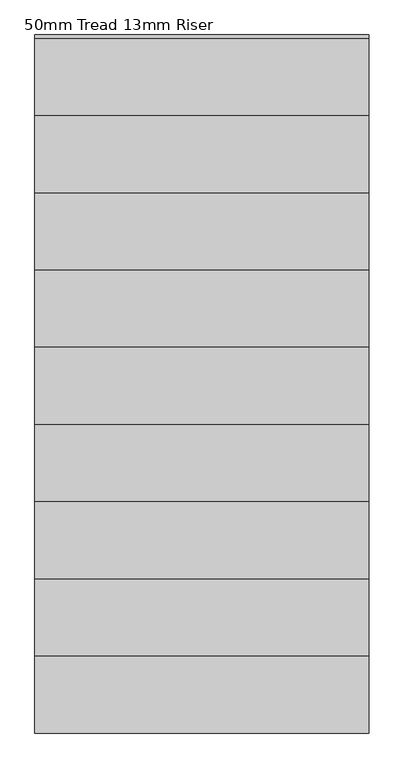
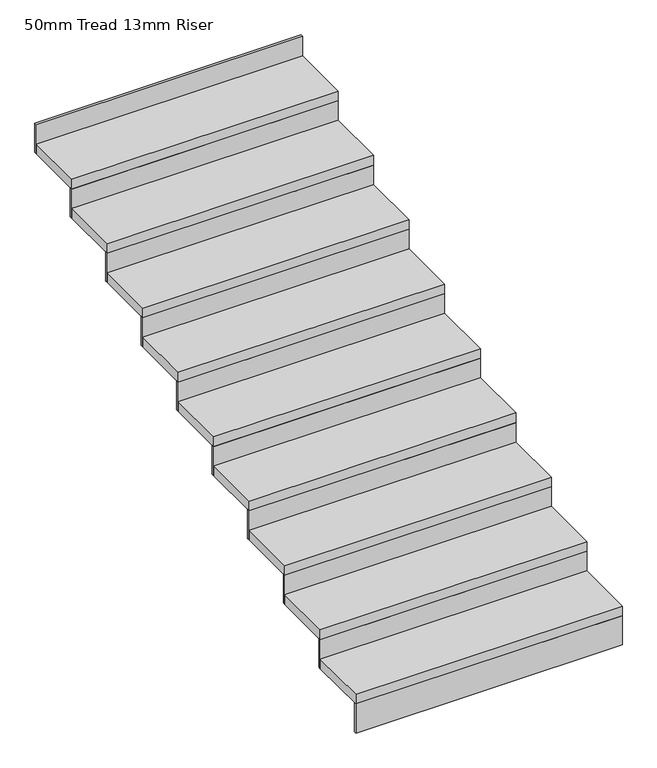
"""IFC4 building model written with IfcOpenShell, lengths in millimetres: stair flight geometry, 50mm Tread 13mm Riser."""

from ifc_helpers import new_model, si_unit, frame, origin, place, context, project, spatial, polyline, outline, extrude, source, transform, mapped, element, save


def stair_flight_50mm_tread_13mm_riser_5745738f(model_context):
    return source(origin(), model_context, "Body", "SweptSolid", [
        extrude(outline(polyline([(-13276.101437, -1587.6378151), (-13276.101437, -1600.1378151), (-14576.101437, -1600.1378151), (-14576.101437, -1587.6378151), (-13276.101437, -1587.6378151)])), frame((0.0, 0.0, 1450.0), z_axis=(0.0, 0.0, 1.0), x_axis=(1.0, 0.0, 0.0)), (0.0, 0.0, 1.0), 150.0),
        extrude(outline(polyline([(-14576.101437, -1300.1378151), (-13276.101437, -1300.1378151), (-13276.101437, -1600.1378151), (-14576.101437, -1600.1378151), (-14576.101437, -1300.1378151)])), frame((0.0, 0.0, 1600.0), z_axis=(0.0, 0.0, 1.0), x_axis=(1.0, 0.0, 0.0)), (0.0, 0.0, 1.0), 50.0),
        extrude(outline(polyline([(-13276.101437, -1287.6378151), (-13276.101437, -1300.1378151), (-14576.101437, -1300.1378151), (-14576.101437, -1287.6378151), (-13276.101437, -1287.6378151)])), frame((0.0, 0.0, 1600.0), z_axis=(0.0, 0.0, 1.0), x_axis=(1.0, 0.0, 0.0)), (0.0, 0.0, 1.0), 150.0),
        extrude(outline(polyline([(-14576.101437, -1000.1378151), (-13276.101437, -1000.1378151), (-13276.101437, -1300.1378151), (-14576.101437, -1300.1378151), (-14576.101437, -1000.1378151)])), frame((0.0, 0.0, 1750.0), z_axis=(0.0, 0.0, 1.0), x_axis=(1.0, 0.0, 0.0)), (0.0, 0.0, 1.0), 50.0),
        extrude(outline(polyline([(-13276.101437, -987.6378151), (-13276.101437, -1000.1378151), (-14576.101437, -1000.1378151), (-14576.101437, -987.6378151), (-13276.101437, -987.6378151)])), frame((0.0, 0.0, 1750.0), z_axis=(0.0, 0.0, 1.0), x_axis=(1.0, 0.0, 0.0)), (0.0, 0.0, 1.0), 150.0),
        extrude(outline(polyline([(-14576.101437, -700.1378151), (-13276.101437, -700.1378151), (-13276.101437, -1000.1378151), (-14576.101437, -1000.1378151), (-14576.101437, -700.1378151)])), frame((0.0, 0.0, 1900.0), z_axis=(0.0, 0.0, 1.0), x_axis=(1.0, 0.0, 0.0)), (0.0, 0.0, 1.0), 50.0),
        extrude(outline(polyline([(-13276.101437, -687.6378151), (-13276.101437, -700.1378151), (-14576.101437, -700.1378151), (-14576.101437, -687.6378151), (-13276.101437, -687.6378151)])), frame((0.0, 0.0, 1900.0), z_axis=(0.0, 0.0, 1.0), x_axis=(1.0, 0.0, 0.0)), (0.0, 0.0, 1.0), 150.0),
        extrude(outline(polyline([(-14576.101437, -400.1378151), (-13276.101437, -400.1378151), (-13276.101437, -700.1378151), (-14576.101437, -700.1378151), (-14576.101437, -400.1378151)])), frame((0.0, 0.0, 2050.0), z_axis=(0.0, 0.0, 1.0), x_axis=(1.0, 0.0, 0.0)), (0.0, 0.0, 1.0), 50.0),
        extrude(outline(polyline([(-13276.101437, -387.6378151), (-13276.101437, -400.1378151), (-14576.101437, -400.1378151), (-14576.101437, -387.6378151), (-13276.101437, -387.6378151)])), frame((0.0, 0.0, 2050.0), z_axis=(0.0, 0.0, 1.0), x_axis=(1.0, 0.0, 0.0)), (0.0, 0.0, 1.0), 150.0),
        extrude(outline(polyline([(-14576.101437, -100.1378151), (-13276.101437, -100.1378151), (-13276.101437, -400.1378151), (-14576.101437, -400.1378151), (-14576.101437, -100.1378151)])), frame((0.0, 0.0, 2200.0), z_axis=(0.0, 0.0, 1.0), x_axis=(1.0, 0.0, 0.0)), (0.0, 0.0, 1.0), 50.0),
        extrude(outline(polyline([(-13276.101437, -87.6378151), (-13276.101437, -100.1378151), (-14576.101437, -100.1378151), (-14576.101437, -87.6378151), (-13276.101437, -87.6378151)])), frame((0.0, 0.0, 2200.0), z_axis=(0.0, 0.0, 1.0), x_axis=(1.0, 0.0, 0.0)), (0.0, 0.0, 1.0), 150.0),
        extrude(outline(polyline([(-14576.101437, 199.8621849), (-13276.101437, 199.8621849), (-13276.101437, -100.1378151), (-14576.101437, -100.1378151), (-14576.101437, 199.8621849)])), frame((0.0, 0.0, 2350.0), z_axis=(0.0, 0.0, 1.0), x_axis=(1.0, 0.0, 0.0)), (0.0, 0.0, 1.0), 50.0),
        extrude(outline(polyline([(-13276.101437, 212.3621849), (-13276.101437, 199.8621849), (-14576.101437, 199.8621849), (-14576.101437, 212.3621849), (-13276.101437, 212.3621849)])), frame((0.0, 0.0, 2350.0), z_axis=(0.0, 0.0, 1.0), x_axis=(1.0, 0.0, 0.0)), (0.0, 0.0, 1.0), 150.0),
        extrude(outline(polyline([(-14576.101437, 499.8621849), (-13276.101437, 499.8621849), (-13276.101437, 199.8621849), (-14576.101437, 199.8621849), (-14576.101437, 499.8621849)])), frame((0.0, 0.0, 2500.0), z_axis=(0.0, 0.0, 1.0), x_axis=(1.0, 0.0, 0.0)), (0.0, 0.0, 1.0), 50.0),
        extrude(outline(polyline([(-13276.101437, 512.3621849), (-13276.101437, 499.8621849), (-14576.101437, 499.8621849), (-14576.101437, 512.3621849), (-13276.101437, 512.3621849)])), frame((0.0, 0.0, 2500.0), z_axis=(0.0, 0.0, 1.0), x_axis=(1.0, 0.0, 0.0)), (0.0, 0.0, 1.0), 150.0),
        extrude(outline(polyline([(-14576.101437, 799.8621849), (-13276.101437, 799.8621849), (-13276.101437, 499.8621849), (-14576.101437, 499.8621849), (-14576.101437, 799.8621849)])), frame((0.0, 0.0, 2650.0), z_axis=(0.0, 0.0, 1.0), x_axis=(1.0, 0.0, 0.0)), (0.0, 0.0, 1.0), 50.0),
        extrude(outline(polyline([(-13276.101437, 812.3621849), (-13276.101437, 799.8621849), (-14576.101437, 799.8621849), (-14576.101437, 812.3621849), (-13276.101437, 812.3621849)])), frame((0.0, 0.0, 2650.0), z_axis=(0.0, 0.0, 1.0), x_axis=(1.0, 0.0, 0.0)), (0.0, 0.0, 1.0), 150.0),
        extrude(outline(polyline([(-13276.101437, 1112.3621849), (-13276.101437, 1099.8621849), (-14576.101437, 1099.8621849), (-14576.101437, 1112.3621849), (-13276.101437, 1112.3621849)])), frame((0.0, 0.0, 2800.0), z_axis=(0.0, 0.0, 1.0), x_axis=(1.0, 0.0, 0.0)), (0.0, 0.0, 1.0), 150.0),
        extrude(outline(polyline([(-14576.101437, 1099.8621849), (-13276.101437, 1099.8621849), (-13276.101437, 799.8621849), (-14576.101437, 799.8621849), (-14576.101437, 1099.8621849)])), frame((0.0, 0.0, 2800.0), z_axis=(0.0, 0.0, 1.0), x_axis=(1.0, 0.0, 0.0)), (0.0, 0.0, 1.0), 50.0),
    ])


if __name__ == "__main__":
    model = new_model("IFC4")
    model_context = context("Model", 3, world=origin())
    ifc_project = project(units=[si_unit("LENGTHUNIT", "METRE", prefix="MILLI")], contexts=[model_context])
    site = spatial("IfcSite", under=ifc_project)
    building = spatial("IfcBuilding", under=site)
    placement = place(None, origin())
    stair_flight_50mm_tread_13mm_riser_shape = stair_flight_50mm_tread_13mm_riser_5745738f(model_context)
    element("IfcStairFlight", 1, ObjectType="50mm Tread 13mm Riser", at=placement, inside=building, context=model_context, shape_type="MappedRepresentation", body=[
        mapped(stair_flight_50mm_tread_13mm_riser_shape, transform((0.0, 0.0, 0.0), x_axis=(1.0, 0.0, 0.0), y_axis=(0.0, 1.0, 0.0), z_axis=(0.0, 0.0, 1.0))),
    ])
    save(model, "model.ifc")
